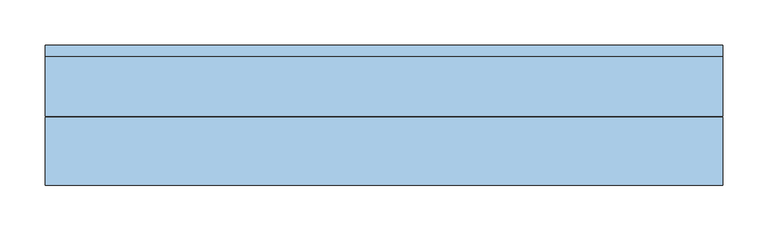
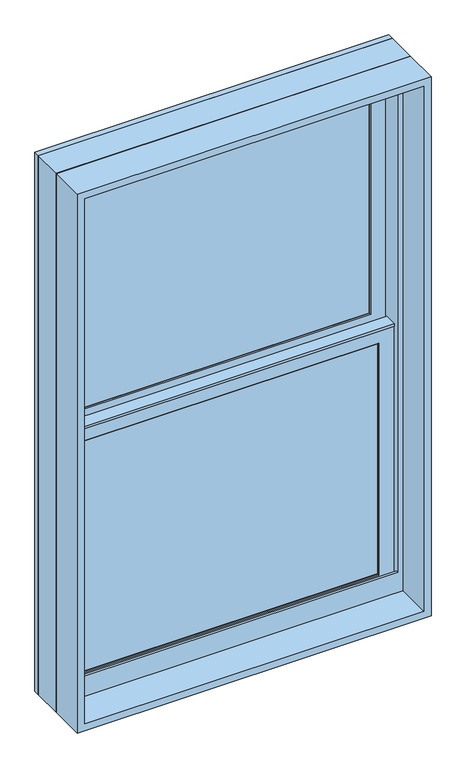
"""IFC4 building model written with IfcOpenShell, lengths in millimetres: window geometry, Window-Double_Hung-Marvin-Essential : ESDH2640."""

from ifc_helpers import new_model, si_unit, frame, origin, place, context, project, spatial, polyline, outline, extrude, faceted_brep, source, transform, mapped, element, save


def window_768a65c7(model_context):
    return source(origin(), model_context, "Body", "SolidModel", [
        extrude(outline(polyline([(115.3583333, 20.6375), (115.3583333, 15.875), (96.3083333, 15.875), (96.3083333, 20.6375), (115.3583333, 20.6375)])), frame((0.0, 0.0, 1289.05), z_axis=(0.0, 0.0, 1.0), x_axis=(1.0, 0.0, 0.0)), (0.0, 0.0, 1.0), 527.05),
        extrude(outline(polyline([(-96.3083333, 20.6375), (-96.3083333, 15.875), (-115.3583333, 15.875), (-115.3583333, 20.6375), (-96.3083333, 20.6375)])), frame((0.0, 0.0, 1289.05), z_axis=(0.0, 0.0, 1.0), x_axis=(1.0, 0.0, 0.0)), (0.0, 0.0, 1.0), 527.05),
        extrude(outline(polyline([(317.5, 20.6375), (317.5, 15.875), (-317.5, 15.875), (-317.5, 20.6375), (317.5, 20.6375)])), frame((0.0, 0.0, 1543.05), z_axis=(0.0, 0.0, 1.0), x_axis=(1.0, 0.0, 0.0)), (0.0, 0.0, 1.0), 19.05),
        extrude(outline(polyline([(-115.3583333, 46.83125), (-115.3583333, 51.59375), (-96.3083333, 51.59375), (-96.3083333, 46.83125), (-115.3583333, 46.83125)])), frame((0.0, 0.0, 1854.2), z_axis=(0.0, 0.0, 1.0), x_axis=(1.0, 0.0, 0.0)), (0.0, 0.0, 1.0), 527.05),
        extrude(outline(polyline([(96.3083333, 46.83125), (96.3083333, 51.59375), (115.3583333, 51.59375), (115.3583333, 46.83125), (96.3083333, 46.83125)])), frame((0.0, 0.0, 1854.2), z_axis=(0.0, 0.0, 1.0), x_axis=(1.0, 0.0, 0.0)), (0.0, 0.0, 1.0), 527.05),
        extrude(outline(polyline([(-317.5, 46.83125), (-317.5, 51.59375), (317.5, 51.59375), (317.5, 46.83125), (-317.5, 46.83125)])), frame((0.0, 0.0, 2108.2), z_axis=(0.0, 0.0, 1.0), x_axis=(1.0, 0.0, 0.0)), (0.0, 0.0, 1.0), 19.05),
        extrude(outline(polyline([(115.3583333, 20.6375), (96.3083333, 20.6375), (96.3083333, 25.4), (115.3583333, 25.4), (115.3583333, 20.6375)])), frame((0.0, 0.0, 1289.05), z_axis=(0.0, 0.0, 1.0), x_axis=(1.0, 0.0, 0.0)), (0.0, 0.0, 1.0), 527.05),
        extrude(outline(polyline([(-96.3083333, 20.6375), (-115.3583333, 20.6375), (-115.3583333, 25.4), (-96.3083333, 25.4), (-96.3083333, 20.6375)])), frame((0.0, 0.0, 1289.05), z_axis=(0.0, 0.0, 1.0), x_axis=(1.0, 0.0, 0.0)), (0.0, 0.0, 1.0), 527.05),
        extrude(outline(polyline([(317.5, 20.6375), (-317.5, 20.6375), (-317.5, 25.4), (317.5, 25.4), (317.5, 20.6375)])), frame((0.0, 0.0, 1543.05), z_axis=(0.0, 0.0, 1.0), x_axis=(1.0, 0.0, 0.0)), (0.0, 0.0, 1.0), 19.05),
        extrude(outline(polyline([(-115.3583333, 56.35625), (-96.3083333, 56.35625), (-96.3083333, 51.59375), (-115.3583333, 51.59375), (-115.3583333, 56.35625)])), frame((0.0, 0.0, 1854.2), z_axis=(0.0, 0.0, 1.0), x_axis=(1.0, 0.0, 0.0)), (0.0, 0.0, 1.0), 527.05),
        extrude(outline(polyline([(96.3083333, 56.35625), (115.3583333, 56.35625), (115.3583333, 51.59375), (96.3083333, 51.59375), (96.3083333, 56.35625)])), frame((0.0, 0.0, 1854.2), z_axis=(0.0, 0.0, 1.0), x_axis=(1.0, 0.0, 0.0)), (0.0, 0.0, 1.0), 527.05),
        extrude(outline(polyline([(-317.5, 56.35625), (317.5, 56.35625), (317.5, 51.59375), (-317.5, 51.59375), (-317.5, 56.35625)])), frame((0.0, 0.0, 2108.2), z_axis=(0.0, 0.0, 1.0), x_axis=(1.0, 0.0, 0.0)), (0.0, 0.0, 1.0), 19.05),
        faceted_brep([(-344.4875, 5.6780605, 1846.1351748), (-344.4875, 5.6780605, 1841.5), (344.4875, 5.6780605, 1841.5), (344.4875, 5.6780605, 1846.1351748), (-344.4875, 34.8118605, 1846.1351748), (344.4875, 34.8118605, 1846.1351748), (344.4875, 34.8118605, 1841.5), (-344.4875, 34.8118605, 1841.5), (-344.4875, 30.1625, 1841.5), (-344.4875, 30.1625, 1262.0625), (-344.4875, 8.9241104, 1262.0625), (-344.4875, 8.9241104, 1841.5), (344.4875, 8.9241104, 1841.5), (344.4875, 30.1625, 1841.5), (344.4875, 8.9241104, 1262.0625), (344.4875, 30.1625, 1262.0625), (-328.6034752, 11.90625, 1827.2034752), (-328.6034752, 30.1625, 1827.2034752), (328.6034752, 30.1625, 1827.2034752), (328.6034752, 11.90625, 1827.2034752), (-311.94375, 10.4662439, 1810.54375), (-311.94375, 11.90625, 1810.54375), (311.94375, 11.90625, 1810.54375), (311.94375, 10.4662439, 1810.54375), (313.4858834, 8.9241104, 1812.0858834), (-313.4858834, 8.9241104, 1812.0858834), (328.6034752, 30.1625, 1277.9465248), (328.6034752, 11.90625, 1277.9465248), (311.94375, 11.90625, 1294.60625), (311.94375, 10.4662439, 1294.60625), (313.4858834, 8.9241104, 1293.0641166), (-328.6034752, 30.1625, 1277.9465248), (-328.6034752, 11.90625, 1277.9465248), (-311.94375, 11.90625, 1294.60625), (-311.94375, 10.4662439, 1294.60625), (-313.4858834, 8.9241104, 1293.0641166)], [[[0, 1, 2, 3]], [[4, 5, 6, 7]], [[1, 0, 4, 7, 8, 9, 10, 11]], [[2, 1, 11, 12]], [[7, 6, 13, 8]], [[3, 2, 12, 14, 15, 13, 6, 5]], [[0, 3, 5, 4]], [[16, 17, 18, 19]], [[20, 21, 22, 23]], [[20, 23, 24, 25]], [[19, 18, 26, 27]], [[23, 22, 28, 29]], [[24, 23, 29, 30]], [[27, 26, 31, 32]], [[29, 28, 33, 34]], [[30, 29, 34, 35]], [[15, 14, 10, 9]], [[15, 9, 8, 13], [18, 17, 31, 26]], [[17, 16, 32, 31]], [[16, 19, 27, 32], [22, 21, 33, 28]], [[21, 20, 34, 33]], [[20, 25, 35, 34]], [[10, 14, 12, 11], [25, 24, 30, 35]]]),
        extrude(outline(polyline([(38.5955581, 1827.2125), (33.5778968, 1827.2125), (33.5778968, 1828.8), (39.9405976, 1828.8), (39.9405976, 1827.2125), (61.515625, 1827.2125), (47.6307501, 1823.8975159), (38.5955581, 1823.8975159), (38.5955581, 1827.2125)])), frame((-344.4875, 0.0, 0.0), z_axis=(1.0, 0.0, 0.0), x_axis=(0.0, 1.0, 0.0)), (0.0, 0.0, 1.0), 688.975),
        faceted_brep([(374.65, 0.0, 1231.9), (374.65, 0.0, 2438.4), (-374.65, 0.0, 2438.4), (-374.65, 0.0, 1231.9), (348.45625, 0.0, 1293.01875), (-348.45625, 0.0, 1293.01875), (-348.45625, 0.0, 2412.20625), (348.45625, 0.0, 2412.20625), (348.45625, 3.96875, 1231.9), (-348.45625, 3.96875, 1231.9), (-348.45625, 3.96875, 1293.01875), (348.45625, 3.96875, 1293.01875), (-374.65, 65.6828125, 1231.9), (-348.45625, 65.6828125, 1231.9), (348.45625, 65.6828125, 1231.9), (374.65, 65.6828125, 1231.9), (-374.65, 65.6828125, 2438.4), (374.65, 65.6828125, 2438.4), (348.45625, 65.6828125, 2412.20625), (-348.45625, 65.6828125, 2412.20625)], [[[0, 1, 2, 3], [4, 5, 6, 7]], [[8, 9, 10, 11]], [[5, 4, 11, 10]], [[0, 3, 12, 13, 9, 8, 14, 15]], [[13, 12, 16, 17, 15, 14, 18, 19]], [[13, 19, 6, 5, 10, 9]], [[7, 6, 19, 18]], [[18, 14, 8, 11, 4, 7]], [[1, 0, 15, 17]], [[2, 1, 17, 16]], [[3, 2, 16, 12]]]),
        faceted_brep([(348.45625, 30.1625, 1835.15), (346.86875, 30.1625, 1835.15), (346.86875, 30.1625, 1256.2544613), (348.45625, 30.1625, 1256.2544613), (-346.86875, 30.1625, 1835.15), (-348.45625, 30.1625, 1835.15), (-348.45625, 30.1625, 1256.2544613), (-346.86875, 30.1625, 1256.2544613), (346.86875, 63.5, 1835.15), (348.45625, 63.5, 1835.15), (348.45625, 63.5, 1249.7743077), (346.86875, 63.5, 1249.7743077), (-348.45625, 63.5, 1835.15), (-346.86875, 63.5, 1835.15), (-346.86875, 63.5, 1249.7743077), (-348.45625, 63.5, 1249.7743077), (359.7108932, 3.96875, 1261.3460105), (359.7108932, 3.96875, 1231.9), (359.7108932, 65.6828125, 1231.9), (359.7108932, 65.6828125, 1249.350012), (-359.7108932, 3.96875, 1231.9), (-359.7108932, 3.96875, 1261.3460105), (-359.7108932, 65.6828125, 1249.350012), (-359.7108932, 65.6828125, 1231.9), (359.7108932, 78.58125, 1246.8428097), (-359.7108932, 78.58125, 1246.8428097), (-357.6971252, 68.2348864, 1248.8539391), (-339.73135, 68.2348864, 1248.8539391), (-339.73135, 65.6828125, 1249.350012), (339.73135, 65.6828125, 1249.350012), (339.73135, 68.2348864, 1248.8539391), (357.6971252, 68.2348864, 1248.8539391), (-374.65, 65.6828125, 1231.9), (-374.65, 78.5948249, 1231.9), (374.65, 78.5948249, 1231.9), (374.65, 65.6828125, 1231.9), (-374.65, 78.58125, 2438.4), (374.65, 78.58125, 2438.4), (359.7108932, 78.58125, 2423.4608932), (-359.7108932, 78.58125, 2423.4608932), (-374.65, 65.6828125, 2438.4), (-357.6971252, 68.2348864, 2421.4471252), (357.6971252, 68.2348864, 2421.4471252), (339.73135, 68.2348864, 2403.48135), (-339.73135, 68.2348864, 2403.48135), (-339.73135, 65.6828125, 2403.48135), (339.73135, 65.6828125, 2403.48135), (374.65, 65.6828125, 2438.4)], [[[0, 1, 2, 3]], [[4, 5, 6, 7]], [[8, 9, 10, 11]], [[12, 13, 14, 15]], [[1, 8, 11, 2]], [[9, 0, 3, 10]], [[1, 0, 9, 8]], [[5, 4, 13, 12]], [[5, 12, 15, 6]], [[13, 4, 7, 14]], [[16, 17, 18, 19]], [[20, 21, 22, 23]], [[24, 25, 26, 27, 28, 22, 21, 16, 19, 29, 30, 31], [3, 2, 11, 10], [7, 6, 15, 14]], [[17, 16, 21, 20]], [[17, 20, 23, 32, 33, 34, 35, 18]], [[34, 33, 36, 37], [25, 24, 38, 39]], [[33, 32, 40, 36]], [[39, 41, 26, 25]], [[41, 42, 31, 30, 43, 44, 27, 26]], [[44, 45, 28, 27]], [[40, 32, 23, 22, 28, 45, 46, 29, 19, 18, 35, 47]], [[36, 40, 47, 37]], [[39, 38, 42, 41]], [[44, 43, 46, 45]], [[34, 37, 47, 35]], [[42, 38, 24, 31]], [[46, 43, 30, 29]]]),
        extrude(outline(polyline([(324.64375, 11.90625), (-324.64375, 11.90625), (-324.64375, 15.08125), (324.64375, 15.08125), (324.64375, 11.90625)])), frame((0.0, 0.0, 1281.90625), z_axis=(0.0, 0.0, 1.0), x_axis=(1.0, 0.0, 0.0)), (0.0, 0.0, 1.0), 541.3375),
        extrude(outline(polyline([(324.64375, 42.8625), (-324.64375, 42.8625), (-324.64375, 46.0375), (324.64375, 46.0375), (324.64375, 42.8625)])), frame((0.0, 0.0, 1847.05625), z_axis=(0.0, 0.0, 1.0), x_axis=(1.0, 0.0, 0.0)), (0.0, 0.0, 1.0), 541.3375),
        faceted_brep([(-311.94375, 31.194477, 1810.54375), (-313.4858834, 32.7366104, 1812.0858834), (313.4858834, 32.7366104, 1812.0858834), (311.94375, 31.194477, 1810.54375), (-311.94375, 30.1625, 1810.54375), (311.94375, 30.1625, 1810.54375), (-344.4875, 32.7366104, 1843.0875), (-344.4875, 30.1625, 1843.0875), (344.4875, 30.1625, 1843.0875), (344.4875, 32.7366104, 1843.0875), (313.4858834, 32.7366104, 1293.0641166), (311.94375, 31.194477, 1294.60625), (311.94375, 30.1625, 1294.60625), (344.4875, 30.1625, 1262.0625), (344.4875, 32.7366104, 1262.0625), (-313.4858834, 32.7366104, 1293.0641166), (-311.94375, 31.194477, 1294.60625), (-311.94375, 30.1625, 1294.60625), (-344.4875, 30.1625, 1262.0625), (-344.4875, 32.7366104, 1262.0625)], [[[0, 1, 2, 3]], [[4, 0, 3, 5]], [[6, 7, 8, 9]], [[3, 2, 10, 11]], [[5, 3, 11, 12]], [[9, 8, 13, 14]], [[11, 10, 15, 16]], [[12, 11, 16, 17]], [[14, 13, 18, 19]], [[9, 14, 19, 6], [1, 15, 10, 2]], [[16, 15, 1, 0]], [[17, 16, 0, 4]], [[7, 18, 13, 8], [5, 12, 17, 4]], [[19, 18, 7, 6]]]),
        faceted_brep([(-328.6034752, 42.8625, 2392.3534752), (-328.6034752, 61.11875, 2392.3534752), (328.6034752, 61.11875, 2392.3534752), (328.6034752, 42.8625, 2392.3534752), (-311.94375, 41.4224939, 2375.69375), (-311.94375, 42.8625, 2375.69375), (311.94375, 42.8625, 2375.69375), (311.94375, 41.4224939, 2375.69375), (-313.4858834, 39.8803604, 2377.2358834), (313.4858834, 39.8803604, 2377.2358834), (-344.4875, 61.11875, 2408.2375), (-344.4875, 39.8803604, 2408.2375), (344.4875, 39.8803604, 2408.2375), (344.4875, 61.11875, 2408.2375), (328.6034752, 61.11875, 1843.0965248), (328.6034752, 42.8625, 1843.0965248), (311.94375, 42.8625, 1859.75625), (311.94375, 41.4224939, 1859.75625), (313.4858834, 39.8803604, 1858.2141166), (344.4875, 39.8803604, 1827.2125), (344.4875, 61.11875, 1827.2125), (-328.6034752, 61.11875, 1843.0965248), (-328.6034752, 42.8625, 1843.0965248), (-311.94375, 42.8625, 1859.75625), (-311.94375, 41.4224939, 1859.75625), (-313.4858834, 39.8803604, 1858.2141166), (-344.4875, 39.8803604, 1827.2125), (-344.4875, 61.11875, 1827.2125)], [[[0, 1, 2, 3]], [[4, 5, 6, 7]], [[8, 4, 7, 9]], [[10, 11, 12, 13]], [[3, 2, 14, 15]], [[7, 6, 16, 17]], [[9, 7, 17, 18]], [[13, 12, 19, 20]], [[15, 14, 21, 22]], [[17, 16, 23, 24]], [[18, 17, 24, 25]], [[20, 19, 26, 27]], [[13, 20, 27, 10], [1, 21, 14, 2]], [[22, 21, 1, 0]], [[3, 15, 22, 0], [5, 23, 16, 6]], [[24, 23, 5, 4]], [[25, 24, 4, 8]], [[11, 26, 19, 12], [9, 18, 25, 8]], [[27, 26, 11, 10]]]),
        faceted_brep([(-344.4875, 61.11875, 1827.2125), (-344.4875, 63.6928604, 1827.2125), (344.4875, 63.6928604, 1827.2125), (344.4875, 61.11875, 1827.2125), (-311.94375, 62.150727, 1859.75625), (-311.94375, 61.11875, 1859.75625), (311.94375, 61.11875, 1859.75625), (311.94375, 62.150727, 1859.75625), (-313.4858834, 63.6928604, 1858.2141166), (313.4858834, 63.6928604, 1858.2141166), (344.4875, 63.6928604, 2408.2375), (344.4875, 61.11875, 2408.2375), (311.94375, 61.11875, 2375.69375), (311.94375, 62.150727, 2375.69375), (313.4858834, 63.6928604, 2377.2358834), (-344.4875, 63.6928604, 2408.2375), (-344.4875, 61.11875, 2408.2375), (-311.94375, 61.11875, 2375.69375), (-311.94375, 62.150727, 2375.69375), (-313.4858834, 63.6928604, 2377.2358834)], [[[0, 1, 2, 3]], [[4, 5, 6, 7]], [[8, 4, 7, 9]], [[3, 2, 10, 11]], [[7, 6, 12, 13]], [[9, 7, 13, 14]], [[11, 10, 15, 16]], [[13, 12, 17, 18]], [[14, 13, 18, 19]], [[16, 15, 1, 0]], [[3, 11, 16, 0], [5, 17, 12, 6]], [[18, 17, 5, 4]], [[19, 18, 4, 8]], [[1, 15, 10, 2], [9, 14, 19, 8]]]),
        extrude(outline(polyline([(324.64375, 26.19375), (-324.64375, 26.19375), (-324.64375, 30.1625), (324.64375, 30.1625), (324.64375, 26.19375)])), frame((0.0, 0.0, 1281.90625), z_axis=(0.0, 0.0, 1.0), x_axis=(1.0, 0.0, 0.0)), (0.0, 0.0, 1.0), 541.3375),
        extrude(outline(polyline([(324.64375, 57.15), (-324.64375, 57.15), (-324.64375, 61.11875), (324.64375, 61.11875), (324.64375, 57.15)])), frame((0.0, 0.0, 1847.05625), z_axis=(0.0, 0.0, 1.0), x_axis=(1.0, 0.0, 0.0)), (0.0, 0.0, 1.0), 541.3375),
        extrude(outline(polyline([(2438.4, 374.65), (2438.4, -374.65), (1231.9, -374.65), (1231.9, 374.65), (2438.4, 374.65)]), holes=[polyline([(2422.525, 358.775), (1247.775, 358.775), (1247.775, -358.775), (2422.525, -358.775), (2422.525, 358.775)])]), frame((0.0, -76.2, 0.0), z_axis=(0.0, 1.0, 0.0), x_axis=(0.0, 0.0, 1.0)), (0.0, 0.0, 1.0), 75.40625),
    ])


if __name__ == "__main__":
    model = new_model("IFC4")
    model_context = context("Model", 3, world=origin())
    ifc_project = project(units=[si_unit("LENGTHUNIT", "METRE", prefix="MILLI")], contexts=[model_context])
    site = spatial("IfcSite", under=ifc_project)
    building = spatial("IfcBuilding", under=site)
    placement = place(None, origin())
    window_shape = window_768a65c7(model_context)
    element("IfcWindow", 1, ObjectType="Window-Double_Hung-Marvin-Essential : ESDH2640", at=placement, inside=building, context=model_context, shape_type="MappedRepresentation", body=[
        mapped(window_shape, transform((0.0, 0.0, 0.0), x_axis=(1.0, 0.0, 0.0), y_axis=(0.0, 1.0, 0.0), z_axis=(0.0, 0.0, 1.0))),
    ])
    save(model, "model.ifc")

# Revit data of these elements
# Type "Window-Double_Hung-Marvin-Essential : ESDH2640"
#   Type Mark = "49"
#   Window Type = "Essential Double Hung"
#   Product data url = "https://bimobject.com/marvin-windows-and-doors/product/marvin-dhwau"
#   Product Guid = "c4a96547-874c-4385-91dc-a058adc19d98"
#   Frame = "All Ultrex"
#   Egress Window = "No"
#   URL = "www.marvin.com"
#   Model = "ESDH2640"
#   Manufacturer = "Marvin Windows and Doors"
#   Label Egress = ""
#   Glass Type = "IG Low E II with Argon"
#   Design Pressure = "DP50"
#   Description = "3048 DBHG"
#   Analytic Construction = "<None>"
#   Prairie Corner Width = 0' - 4"
#   Prairie Corner Height = 0' - 4"
#   Egress Width = 2' - 2 9/16"
#   Egress Height = 1' - 7 27/128"
#   Rough Width = 2' - 6"
#   Rough Height = 4' - 0"
#   Nominal Width = 2' - 6"
#   Nominal Height = 4' - 0"
#   Inset to Installation Flange [instance default] = 0' - 1"
#   Height = 3' - 11 1/2"
#   Egress Area = 3.54368 SF
#   Default Head Height = 8' - 0"
#   Width = 2' - 5 1/2"
#   Daylight Area = 6.92952 SF
#   DLO Width = 2' - 0 9/16"
#   DLO Height = 1' - 8 5/16"
#   Muntins Top Sash = yes
#   Lites Wide Top Sash = 3
#   Lites Wide Bottom Sash = 3
#   Lites High Top Sash = 2
#   Lites High Bottom Sash = 2
#   Lite Cut Prairie 9 = no
#   Lite Cut HV Grid = yes
#   Muntins Bottom Sash = yes
#   Label Visibility = no
#   Jamb Extension Visibility = yes
#   Edition number = 1
#   Interior Material = Ultrex-Marvin-Stonewhite
#   Glazing Material = Glass-Marvin-IG Low E II with Argon
#   Cladding Material = Ultrex-Marvin-Pebblegray
#   Wall Closure = (empty or 0)
#   Assembly Code = ""
# Element 1 (IfcWindow, "Window-Double_Hung-Marvin-Essential : ESDH2640")
#   Materials on its faces: "Ultrex-Marvin-Pebblegray", "Ultrex-Marvin-Stonewhite", "Glass-Marvin-IG Low E II with Argon"
# Materials
#   "Ultrex-Marvin-Stonewhite": class "Paint", colour RGB 250 251 245, transparency 0
#   "Glass-Marvin-IG Low E II with Argon": class "Glass", colour RGB 0 128 192, transparency 0.85
#   "Ultrex-Marvin-Pebblegray": class "Paint", colour RGB 189 185 173, transparency 0
